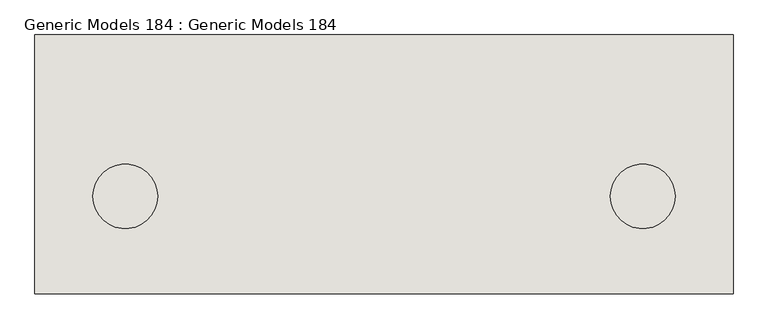
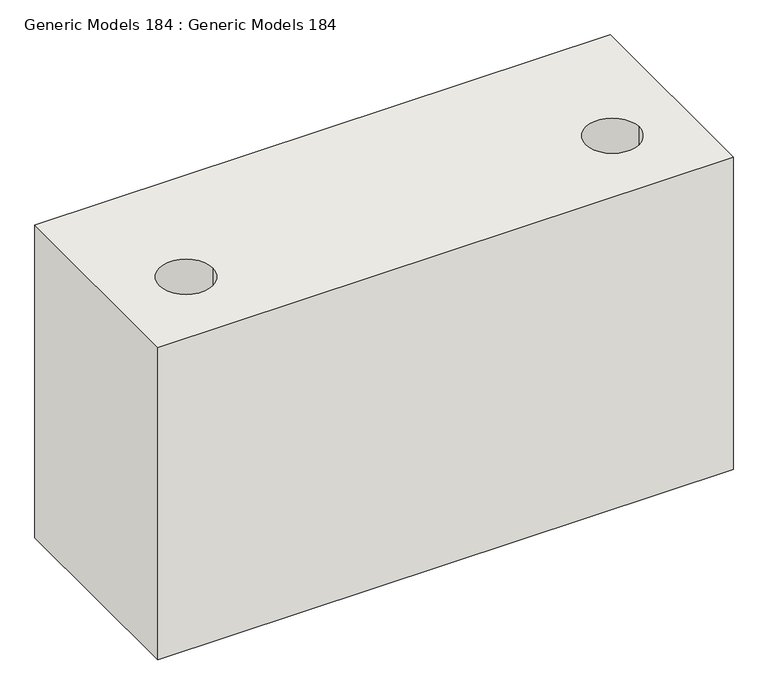
"""IFC4 building model written with IfcOpenShell, lengths in millimetres: wall geometry, Generic Models 184 : Generic Models 184."""

from ifc_helpers import new_model, si_unit, frame, origin, place, context, project, spatial, polyline, circle_curve, source, transform, mapped, element, save
from ifc_brep_helpers import plane_surface, revolved_surface, advanced_brep


def generic_models_184_generic_models_184_bac2a47e(model_context):
    return source(origin(), model_context, "Body", "AdvancedBrep", [
        advanced_brep(
        [(57021.4125, 1219.2, -23.9117188), (53732.1125, 1219.2, -23.9117188), (53732.1125, 0.0, -23.9117188), (57021.4125, 0.0, -23.9117188), (56443.5625, 458.7875, -23.9117188), (56748.3625, 458.7875, -23.9117188), (54005.1625, 458.7875, -23.9117188), (54309.9625, 458.7875, -23.9117188), (57021.4125, 1219.2, -1915.3720904), (57021.4125, 0.0, -1915.3720904), (53732.1125, 0.0, -1915.3720904), (53732.1125, 1219.2, -1915.3720904), (56443.5625, 458.7875, -1219.2), (56748.3625, 458.7875, -1219.2), (54005.1625, 458.7875, -1219.2), (54309.9625, 458.7875, -1219.2)],
        [
            (0, 1),
            (1, 2),
            (2, 3),
            (3, 0),
            (4, 5, circle_curve(frame((56595.9625, 458.7875, -23.9117188), z_axis=(0.0, 0.0, -1.0), x_axis=(1.0, 0.0, 0.0)), 152.4)),
            (5, 4, circle_curve(frame((56595.9625, 458.7875, -23.9117188), z_axis=(0.0, 0.0, -1.0), x_axis=(1.0, 0.0, 0.0)), 152.4)),
            (6, 7, circle_curve(frame((54157.5625, 458.7875, -23.9117188), z_axis=(0.0, 0.0, -1.0), x_axis=(1.0, 0.0, 0.0)), 152.4)),
            (7, 6, circle_curve(frame((54157.5625, 458.7875, -23.9117188), z_axis=(0.0, 0.0, -1.0), x_axis=(1.0, 0.0, 0.0)), 152.4)),
            (8, 9),
            (9, 10),
            (10, 11),
            (11, 8),
            (0, 8),
            (11, 1),
            (10, 2),
            (9, 3),
            (12, 13, circle_curve(frame((56595.9625, 458.7875, -1219.2), z_axis=(0.0, 0.0, 1.0), x_axis=(1.0, 0.0, 0.0)), 152.4)),
            (13, 12, circle_curve(frame((56595.9625, 458.7875, -1219.2), z_axis=(0.0, 0.0, 1.0), x_axis=(1.0, 0.0, 0.0)), 152.4)),
            (14, 15, circle_curve(frame((54157.5625, 458.7875, -1219.2), z_axis=(0.0, 0.0, 1.0), x_axis=(1.0, 0.0, 0.0)), 152.4)),
            (15, 14, circle_curve(frame((54157.5625, 458.7875, -1219.2), z_axis=(0.0, 0.0, 1.0), x_axis=(1.0, 0.0, 0.0)), 152.4)),
            (13, 5),
            (4, 12),
            (15, 7),
            (6, 14),
        ],
        [
            plane_surface(frame((53732.1125, 1219.2, -23.9117188), z_axis=(0.0, 0.0, 1.0), x_axis=(-1.0, 0.0, 0.0))),
            plane_surface(frame((53732.1125, 1219.2, -1915.3720904), z_axis=(0.0, 0.0, -1.0), x_axis=(1.0, 0.0, 0.0))),
            plane_surface(frame((57021.4125, 1219.2, -23.9117188), z_axis=(0.0, 1.0, 0.0), x_axis=(0.0, 0.0, -1.0))),
            plane_surface(frame((53732.1125, 1219.2, -23.9117188), z_axis=(-1.0, 0.0, 0.0), x_axis=(0.0, 0.0, -1.0))),
            plane_surface(frame((53732.1125, 0.0, -23.9117188), z_axis=(0.0, -1.0, 0.0), x_axis=(0.0, 0.0, -1.0))),
            plane_surface(frame((57021.4125, 0.0, -23.9117188), z_axis=(1.0, 0.0, 0.0), x_axis=(0.0, 0.0, -1.0))),
            plane_surface(frame((56748.3625, 458.7875, -1219.2), z_axis=(0.0, 0.0, 1.0), x_axis=(0.0, -1.0, 0.0))),
            revolved_surface(polyline([(56748.3625, 458.7875, -23.911718800000017), (56748.3625, 458.7875, -1219.2)]), (56595.9625, 458.7875, -1219.2), (0.0, 0.0, 1.0)),
            revolved_surface(polyline([(54309.9625, 458.7875, -23.9117188), (54309.9625, 458.7875, -1219.2)]), (54157.5625, 458.7875, 0.0), (0.0, 0.0, 1.0)),
        ],
        [
            (0, [[1, 2, 3, 4], [5, 6], [7, 8]]),
            (1, [[9, 10, 11, 12]]),
            (2, [[-1, 13, -12, 14]]),
            (3, [[-2, -14, -11, 15]]),
            (4, [[-3, -15, -10, 16]]),
            (5, [[-4, -16, -9, -13]]),
            (6, [[17, 18]]),
            (6, [[19, 20]]),
            (7, [[-18, 21, -5, 22]]),
            (7, [[-17, -22, -6, -21]]),
            (8, [[-20, 23, -7, 24]]),
            (8, [[-19, -24, -8, -23]]),
        ],
    ),
    ])


if __name__ == "__main__":
    model = new_model("IFC4")
    model_context = context("Model", 3, world=origin())
    ifc_project = project(units=[si_unit("LENGTHUNIT", "METRE", prefix="MILLI")], contexts=[model_context])
    site = spatial("IfcSite", under=ifc_project)
    building = spatial("IfcBuilding", under=site)
    placement = place(None, origin())
    generic_models_184_generic_models_184_shape = generic_models_184_generic_models_184_bac2a47e(model_context)
    element("IfcWall", 1, ObjectType="Generic Models 184 : Generic Models 184", at=placement, inside=building, context=model_context, shape_type="MappedRepresentation", body=[
        mapped(generic_models_184_generic_models_184_shape, transform((0.0, 0.0, 0.0), x_axis=(1.0, 0.0, 0.0), y_axis=(0.0, 1.0, 0.0), z_axis=(0.0, 0.0, 1.0))),
    ])
    save(model, "model.ifc")

# Revit data of these elements
# Element 1 (IfcWall, "Generic Models 184 : Generic Models 184")
#   Materials on its faces: "GRADE"
# Materials
#   "GRADE": class "Generic", colour RGB 255 255 255, transparency 0, Description = "Soil", Cost = 0
